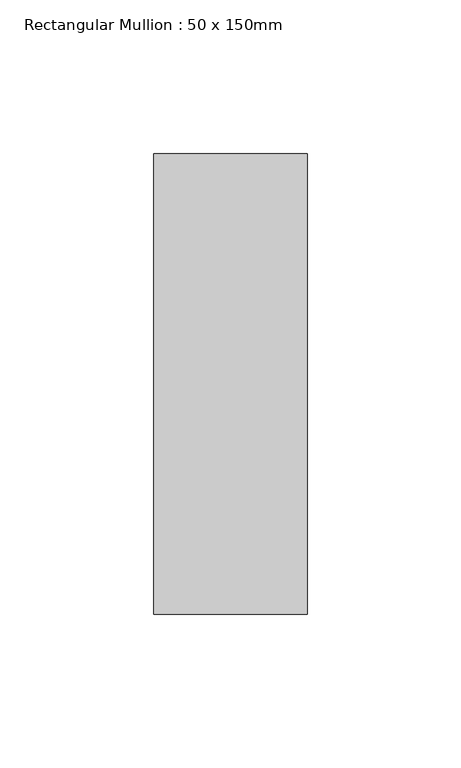
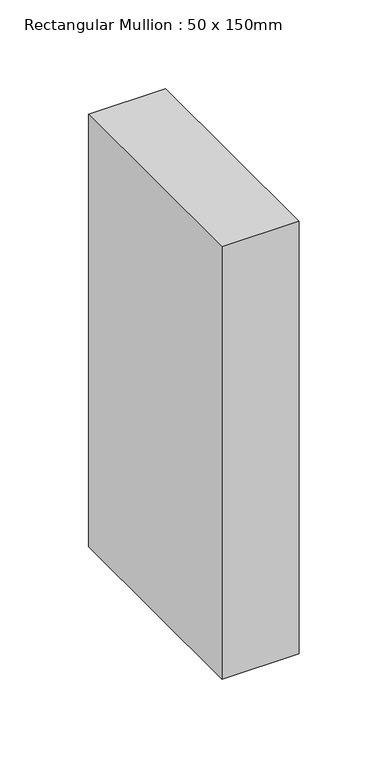
"""IFC4 building model written with IfcOpenShell, lengths in millimetres: member geometry, Rectangular Mullion : 50 x 150mm."""

from ifc_helpers import new_model, si_unit, frame, origin, place, context, project, spatial, polyline, outline, extrude, source, transform, mapped, element, save


def rectangular_mullion_50_x_150mm_7132327f(model_context):
    return source(origin(), model_context, "Body", "SweptSolid", [
        extrude(outline(polyline([(0.0, 75.0), (0.0, -75.0), (-50.0, -75.0), (-50.0, 75.0), (0.0, 75.0)])), frame((0.0, 0.0, -296.7839703), z_axis=(0.0, 0.0, 1.0), x_axis=(1.0, 0.0, 0.0)), (0.0, 0.0, 1.0), 296.7839703),
    ])


if __name__ == "__main__":
    model = new_model("IFC4")
    model_context = context("Model", 3, world=origin())
    ifc_project = project(units=[si_unit("LENGTHUNIT", "METRE", prefix="MILLI")], contexts=[model_context])
    site = spatial("IfcSite", under=ifc_project)
    building = spatial("IfcBuilding", under=site)
    placement = place(None, origin())
    rectangular_mullion_50_x_150mm_shape = rectangular_mullion_50_x_150mm_7132327f(model_context)
    element("IfcMember", 1, ObjectType="Rectangular Mullion : 50 x 150mm", at=placement, inside=building, context=model_context, shape_type="MappedRepresentation", body=[
        mapped(rectangular_mullion_50_x_150mm_shape, transform((0.0, 0.0, 0.0), x_axis=(1.0, 0.0, 0.0), y_axis=(0.0, 1.0, 0.0), z_axis=(0.0, 0.0, 1.0))),
    ])
    save(model, "model.ifc")

# Revit data of these elements
# Type "Rectangular Mullion : 50 x 150mm"
#   built-in parameter 1007304 = 0.492126 (stored number, unit not read)
#   built-in parameter 1007301 = 0.082021 (stored number, unit not read)
#   built-in parameter 1007300 = 0.082021 (stored number, unit not read)
# Element 1 (IfcMember, "Rectangular Mullion : 50 x 150mm")
#   Materials on its faces: "Aluminium"
# Materials
#   "Aluminium": class "Metal", colour RGB 247 247 247, transparency 0, Description = "Aluminium 6061", Cost = 0
